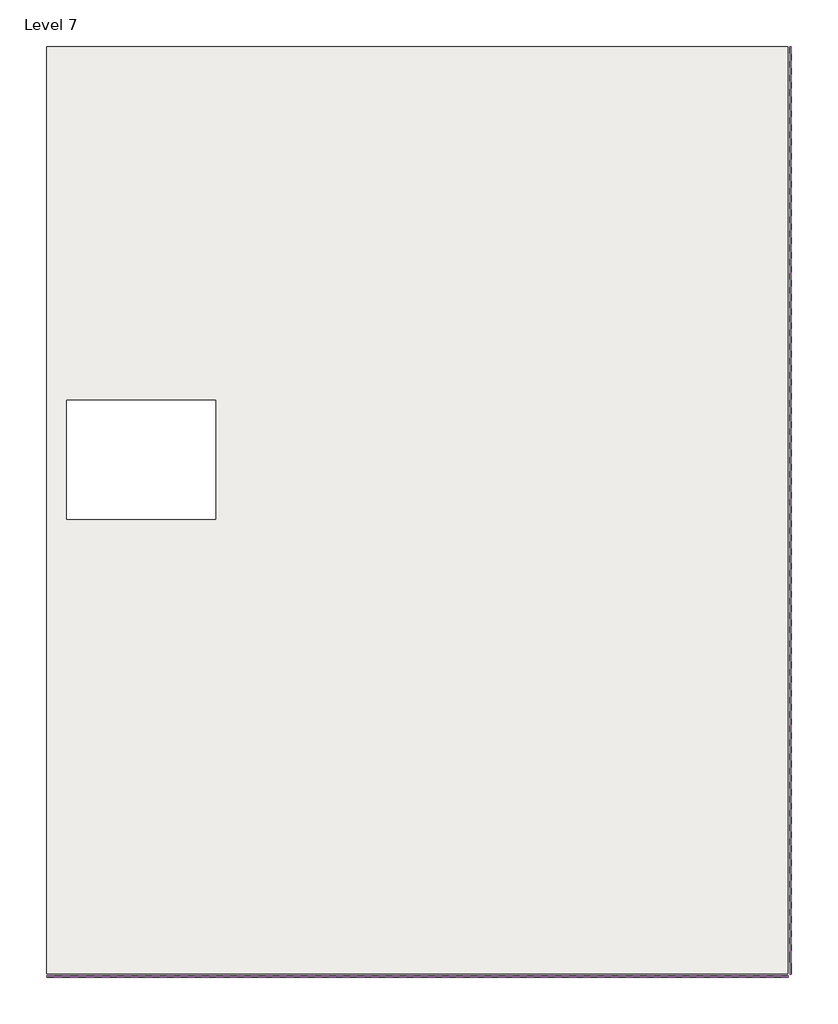
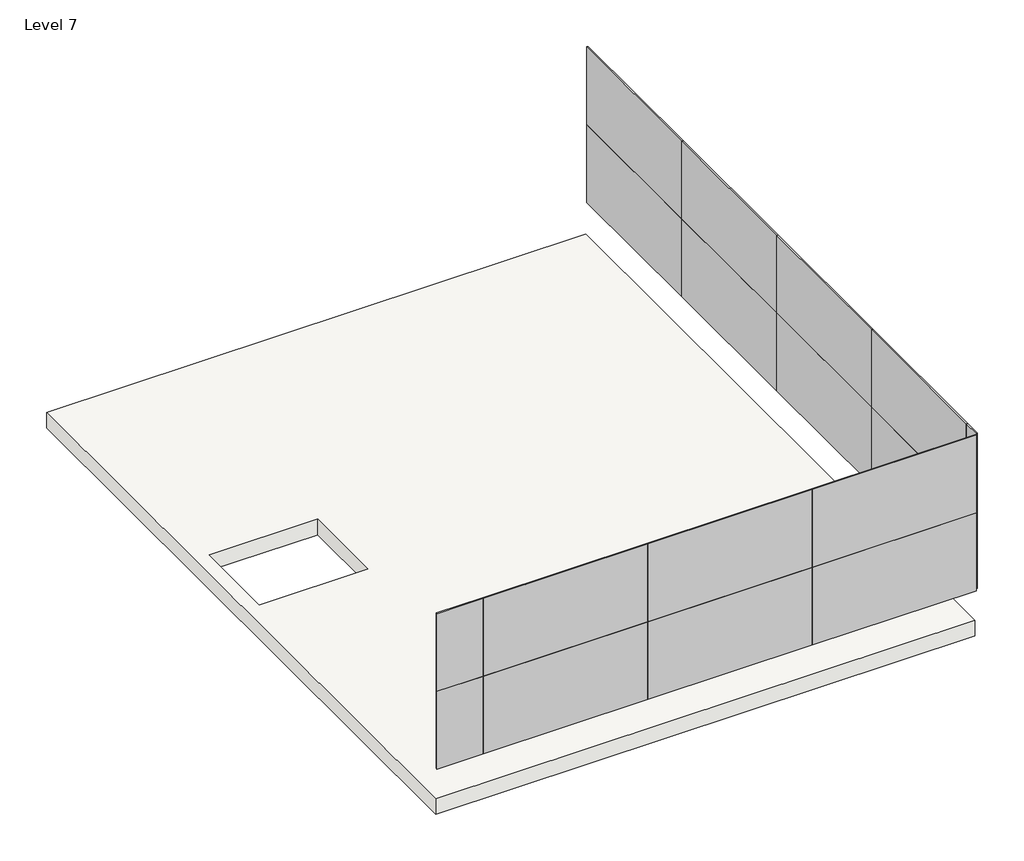
# One storey: 18 plates, 1 slab.
"""IFC4 building model written with IfcOpenShell, lengths in millimetres."""

import ifcopenshell
import ifcopenshell.guid

model = None  # the IFC model being written
_history = None  # IfcOwnerHistory: only IFC2X3 demands one
_inside = {}  # id of a spatial element -> (the spatial element, [elements in it])
_under = {}  # id of a project, library or spatial element -> (it, [spatial elements below it])
_declared = {}  # id of a project -> (the project, [libraries it declares])
_typed = {}  # id of a type object -> (the type object, [elements of that type])
_made_of = {}  # id of a material, layer set ... -> (it, [elements and type objects made of it])


def new_model(schema):
    """Start an empty IFC model of exactly this schema.

    Asked for "IFC4X3", IfcOpenShell would pick the latest addendum, in which some entities
    have other attributes; the version numbers below select the first issue.
    IFC2X3 requires an IfcOwnerHistory on every rooted entity: one is made here for all.
    """
    global model, _history
    if schema == "IFC4X3":
        model = ifcopenshell.file(schema_version=(4, 3, 0, 0))
    else:
        model = ifcopenshell.file(schema=schema)
    _inside.clear()
    _under.clear()
    _declared.clear()
    _typed.clear()
    _made_of.clear()
    _history = None
    if model.schema == "IFC2X3":
        org = make("IfcOrganization", Name="unknown")
        user = make(
            "IfcPersonAndOrganization",
            ThePerson=make("IfcPerson", FamilyName="unknown"),
            TheOrganization=org,
        )
        app = make(
            "IfcApplication",
            ApplicationDeveloper=org,
            Version="unknown",
            ApplicationFullName="unknown",
            ApplicationIdentifier="unknown",
        )
        _history = make(
            "IfcOwnerHistory",
            OwningUser=user,
            OwningApplication=app,
            ChangeAction="ADDED",
            CreationDate=0,
        )
    return model


def make(cls, **values):
    """One entity of the class cls with the attributes given. An attribute that is None is left unset."""
    return model.create_entity(
        cls, **{name: value for name, value in values.items() if value is not None}
    )


def rooted(cls, **values):
    """An entity with a GlobalId (a new one), such as an element, a storey or a relation."""
    return make(cls, GlobalId=ifcopenshell.guid.new(), OwnerHistory=_history, **values)


def si_unit(unit_type, name, prefix=None):
    """IfcSIUnit, for example si_unit("LENGTHUNIT", "METRE", prefix="MILLI")."""
    return make("IfcSIUnit", UnitType=unit_type, Prefix=prefix, Name=name)


def assignment(units):
    """IfcUnitAssignment: the units of a project."""
    return None if units is None else make("IfcUnitAssignment", Units=units)


def point(xyz):
    """IfcCartesianPoint."""
    return None if xyz is None else make("IfcCartesianPoint", Coordinates=xyz)


def direction(xyz):
    """IfcDirection."""
    return None if xyz is None else make("IfcDirection", DirectionRatios=xyz)


def frame(location, z_axis=None, x_axis=None):
    """IfcAxis2Placement3D, a coordinate frame: its origin and axes. An axis left out is left unset."""
    return make(
        "IfcAxis2Placement3D",
        Location=point(location),
        Axis=direction(z_axis),
        RefDirection=direction(x_axis),
    )


def origin():
    """The frame at (0, 0, 0) with its axes left unset."""
    return frame((0.0, 0.0, 0.0))


def origin_with_axes():
    """The frame at (0, 0, 0) with the z axis (0, 0, 1) and the x axis (1, 0, 0) written out."""
    return frame((0.0, 0.0, 0.0), z_axis=(0.0, 0.0, 1.0), x_axis=(1.0, 0.0, 0.0))


def place(relative_to, where):
    """IfcLocalPlacement: puts the frame where relative to a parent placement (None: the world)."""
    return make(
        "IfcLocalPlacement", PlacementRelTo=relative_to, RelativePlacement=where
    )


def context(
    kind, dimensions, precision=None, world=None, true_north=None, identifier=None
):
    """IfcGeometricRepresentationContext, for example the 3D "Model" context."""
    return make(
        "IfcGeometricRepresentationContext",
        ContextIdentifier=identifier,
        ContextType=kind,
        CoordinateSpaceDimension=dimensions,
        Precision=precision,
        WorldCoordinateSystem=world,
        TrueNorth=true_north,
    )


def project(units=None, contexts=None):
    """IfcProject with its units and contexts."""
    return rooted(
        "IfcProject",
        Name="project",
        RepresentationContexts=contexts,
        UnitsInContext=assignment(units),
    )


def spatial(cls, under=None, at=None, **own):
    """A site, building, storey or space (cls), placed at a placement, below another one or the project."""
    s = rooted(cls, ObjectPlacement=at, **own)
    if under is not None:
        _under.setdefault(under.id(), (under, []))[1].append(s)
    return s


def polyline(points):
    """IfcPolyline through the points."""
    return make("IfcPolyline", Points=[point(p) for p in points])


def outline(outer, holes=None, kind="AREA"):
    """IfcArbitraryClosedProfileDef: a profile drawn as a closed curve; with holes, ...WithVoids."""
    if holes is None:
        return make("IfcArbitraryClosedProfileDef", ProfileType=kind, OuterCurve=outer)
    return make(
        "IfcArbitraryProfileDefWithVoids",
        ProfileType=kind,
        OuterCurve=outer,
        InnerCurves=holes,
    )


def extrude(swept, where, along, depth):
    """IfcExtrudedAreaSolid: the profile swept, set in the frame where, extruded along a direction by depth."""
    return make(
        "IfcExtrudedAreaSolid",
        SweptArea=swept,
        Position=where,
        ExtrudedDirection=direction(along),
        Depth=depth,
    )


def shape(context_of_items, identifier, shape_type, items):
    """IfcShapeRepresentation: the items that make up one representation, for example the "Body"."""
    return make(
        "IfcShapeRepresentation",
        ContextOfItems=context_of_items,
        RepresentationIdentifier=identifier,
        RepresentationType=shape_type,
        Items=items,
    )


def source(mapping_origin, context_of_items, identifier, shape_type, items):
    """IfcRepresentationMap: a shape defined once, which mapped items show again and again."""
    return make(
        "IfcRepresentationMap",
        MappingOrigin=mapping_origin,
        MappedRepresentation=shape(context_of_items, identifier, shape_type, items),
    )


def transform(
    local_origin,
    x_axis=None,
    y_axis=None,
    z_axis=None,
    scale=None,
    scale2=None,
    scale3=None,
    uniform=True,
):
    """IfcCartesianTransformationOperator3D, or its non-uniform kind. x_axis, y_axis, z_axis: its Axis1, 2, 3."""
    if uniform:
        return make(
            "IfcCartesianTransformationOperator3D",
            Axis1=direction(x_axis),
            Axis2=direction(y_axis),
            LocalOrigin=point(local_origin),
            Scale=scale,
            Axis3=direction(z_axis),
        )
    return make(
        "IfcCartesianTransformationOperator3DnonUniform",
        Axis1=direction(x_axis),
        Axis2=direction(y_axis),
        LocalOrigin=point(local_origin),
        Scale=scale,
        Axis3=direction(z_axis),
        Scale2=scale2,
        Scale3=scale3,
    )


def mapped(mapping_source, mapping_target):
    """IfcMappedItem: shows the shape of a source again, moved by a transform."""
    return make(
        "IfcMappedItem", MappingSource=mapping_source, MappingTarget=mapping_target
    )


def made_of(thing, what):
    """Note that an element or type object is made of a material, layer set ...; save() writes the relation."""
    if what is not None:
        _made_of.setdefault(what.id(), (what, []))[1].append(thing)
    return thing


def element(
    cls,
    number,
    at=None,
    inside=None,
    cuts=None,
    type_object=None,
    material=None,
    context=None,
    identifier="Body",
    shape_type=None,
    held_by="IfcProductDefinitionShape",
    body=None,
    shapes=None,
    **own,
):
    """One element of the class cls, such as IfcWall. Its Tag is "e" and its number.

    at: its placement. inside: the storey or other place that contains it. cuts: it is an
    opening in that element (IfcRelVoidsElement). A single representation is given by context,
    identifier, shape_type and body (its items); several are given by shapes. held_by: the class
    of the entity that holds the representations. save() writes the other relations.
    """
    e = rooted(cls, Tag="e%d" % number, ObjectPlacement=at, **own)
    if body is not None:
        shapes = [shape(context, identifier, shape_type, body)]
    if shapes is not None:
        e.Representation = make(held_by, Representations=shapes)
    if inside is not None:
        _inside.setdefault(inside.id(), (inside, []))[1].append(e)
    if cuts is not None:
        rooted(
            "IfcRelVoidsElement", RelatingBuildingElement=cuts, RelatedOpeningElement=e
        )
    if type_object is not None:
        _typed.setdefault(type_object.id(), (type_object, []))[1].append(e)
    return made_of(e, material)


def aggregate(whole, parts):
    """IfcRelAggregates: a whole, such as a stair, and the parts it consists of."""
    return rooted("IfcRelAggregates", RelatingObject=whole, RelatedObjects=parts)


def save(model, path):
    """Write the relations noted so far, then the file.

    IfcRelAggregates (storeys below a building ...), IfcRelContainedInSpatialStructure (elements
    in a storey), IfcRelDefinesByType, IfcRelAssociatesMaterial and IfcRelDeclares: one each for
    every whole, place, type object, material and project.
    """
    for whole, parts in _under.values():
        aggregate(whole, parts)
    for where, things in _inside.values():
        rooted(
            "IfcRelContainedInSpatialStructure",
            RelatedElements=things,
            RelatingStructure=where,
        )
    for kind, things in _typed.values():
        rooted("IfcRelDefinesByType", RelatedObjects=things, RelatingType=kind)
    for what, things in _made_of.values():
        rooted("IfcRelAssociatesMaterial", RelatedObjects=things, RelatingMaterial=what)
    for by, libraries in _declared.values():
        rooted("IfcRelDeclares", RelatingContext=by, RelatedDefinitions=libraries)
    model.write(path)


def system_panel_glazed_1e57f9bb(model_context):
    return source(origin(), model_context, "Body", "SweptSolid", [
        extrude(outline(polyline([(1524.0000002, 19.05), (-1524.0000002, 19.05), (-1524.0000002, 44.45), (1524.0000002, 44.45), (1524.0000002, 19.05)])), origin_with_axes(), (0.0, 0.0, 1.0), 1524.0),
    ])


def system_panel_glazed_ccfd9adb(model_context):
    return source(origin(), model_context, "Body", "SweptSolid", [
        extrude(outline(polyline([(427.9999998, 19.05), (-427.9999998, 19.05), (-427.9999998, 44.45), (427.9999998, 44.45), (427.9999998, 19.05)])), origin_with_axes(), (0.0, 0.0, 1.0), 1524.0),
    ])


def system_panel_glazed_88f24eba(model_context):
    return source(origin(), model_context, "Body", "SweptSolid", [
        extrude(outline(polyline([(153.9999998, 19.05), (-153.9999998, 19.05), (-153.9999998, 44.45), (153.9999998, 44.45), (153.9999998, 19.05)])), origin_with_axes(), (0.0, 0.0, 1.0), 1524.0),
    ])


model = new_model("IFC4")

# Units and contexts
model_context = context("Model", 3, world=origin())
ifc_project = project(units=[si_unit("LENGTHUNIT", "METRE", prefix="MILLI")], contexts=[model_context])

# Site, building, storey
site = spatial("IfcSite", under=ifc_project)
building = spatial("IfcBuilding", under=site)
storey = spatial("IfcBuildingStorey", under=building, Name="Level 7", Elevation=19200.0)

# Plates
placement = place(None, origin())
system_panel_glazed_shape = system_panel_glazed_1e57f9bb(model_context)
element("IfcPlate", 1, ObjectType="System Panel : Glazed", at=placement, inside=storey, context=model_context, shape_type="MappedRepresentation", body=[
    mapped(system_panel_glazed_shape, transform((2137.6340362, 1399.6955828, 19812.0), x_axis=(-1.0, 0.0, 0.0), y_axis=(0.0, -1.0, 0.0), z_axis=(0.0, 0.0, 1.0))),
])
element("IfcPlate", 2, ObjectType="System Panel : Glazed", at=placement, inside=storey, context=model_context, shape_type="MappedRepresentation", body=[
    mapped(system_panel_glazed_shape, transform((-910.3659639, 1399.6955828, 19812.0), x_axis=(-1.0, 0.0, 0.0), y_axis=(0.0, -1.0, 0.0), z_axis=(0.0, 0.0, 1.0))),
])
element("IfcPlate", 3, ObjectType="System Panel : Glazed", at=placement, inside=storey, context=model_context, shape_type="MappedRepresentation", body=[
    mapped(system_panel_glazed_shape, transform((-3958.3659639, 1399.6955828, 19812.0), x_axis=(-1.0, 0.0, 0.0), y_axis=(0.0, -1.0, 0.0), z_axis=(0.0, 0.0, 1.0))),
])
element("IfcPlate", 4, ObjectType="System Panel : Glazed", at=placement, inside=storey, context=model_context, shape_type="MappedRepresentation", body=[
    mapped(system_panel_glazed_shape, transform((2137.6340362, 1399.6955828, 21336.0), x_axis=(-1.0, 0.0, 0.0), y_axis=(0.0, -1.0, 0.0), z_axis=(0.0, 0.0, 1.0))),
])
element("IfcPlate", 5, ObjectType="System Panel : Glazed", at=placement, inside=storey, context=model_context, shape_type="MappedRepresentation", body=[
    mapped(system_panel_glazed_shape, transform((-910.3659639, 1399.6955828, 21336.0), x_axis=(-1.0, 0.0, 0.0), y_axis=(0.0, -1.0, 0.0), z_axis=(0.0, 0.0, 1.0))),
])
element("IfcPlate", 6, ObjectType="System Panel : Glazed", at=placement, inside=storey, context=model_context, shape_type="MappedRepresentation", body=[
    mapped(system_panel_glazed_shape, transform((-3958.3659639, 1399.6955828, 21336.0), x_axis=(-1.0, 0.0, 0.0), y_axis=(0.0, -1.0, 0.0), z_axis=(0.0, 0.0, 1.0))),
])
element("IfcPlate", 7, ObjectType="System Panel : Glazed", at=placement, inside=storey, context=model_context, shape_type="MappedRepresentation", body=[
    mapped(system_panel_glazed_shape, transform((3661.6340364, 12375.6955827, 19812.0), x_axis=(0.0, -1.0, 0.0), y_axis=(1.0, 0.0, 0.0), z_axis=(0.0, 0.0, 1.0))),
])
element("IfcPlate", 8, ObjectType="System Panel : Glazed", at=placement, inside=storey, context=model_context, shape_type="MappedRepresentation", body=[
    mapped(system_panel_glazed_shape, transform((3661.6340364, 9327.6955825, 19812.0), x_axis=(0.0, -1.0, 0.0), y_axis=(1.0, 0.0, 0.0), z_axis=(0.0, 0.0, 1.0))),
])
element("IfcPlate", 9, ObjectType="System Panel : Glazed", at=placement, inside=storey, context=model_context, shape_type="MappedRepresentation", body=[
    mapped(system_panel_glazed_shape, transform((3661.6340364, 6279.6955825, 19812.0), x_axis=(0.0, -1.0, 0.0), y_axis=(1.0, 0.0, 0.0), z_axis=(0.0, 0.0, 1.0))),
])
element("IfcPlate", 10, ObjectType="System Panel : Glazed", at=placement, inside=storey, context=model_context, shape_type="MappedRepresentation", body=[
    mapped(system_panel_glazed_shape, transform((3661.6340364, 3231.6955825, 19812.0), x_axis=(0.0, -1.0, 0.0), y_axis=(1.0, 0.0, 0.0), z_axis=(0.0, 0.0, 1.0))),
])
element("IfcPlate", 11, ObjectType="System Panel : Glazed", at=placement, inside=storey, context=model_context, shape_type="MappedRepresentation", body=[
    mapped(system_panel_glazed_shape, transform((3661.6340364, 12375.6955827, 21336.0), x_axis=(0.0, -1.0, 0.0), y_axis=(1.0, 0.0, 0.0), z_axis=(0.0, 0.0, 1.0))),
])
element("IfcPlate", 12, ObjectType="System Panel : Glazed", at=placement, inside=storey, context=model_context, shape_type="MappedRepresentation", body=[
    mapped(system_panel_glazed_shape, transform((3661.6340364, 9327.6955825, 21336.0), x_axis=(0.0, -1.0, 0.0), y_axis=(1.0, 0.0, 0.0), z_axis=(0.0, 0.0, 1.0))),
])
element("IfcPlate", 13, ObjectType="System Panel : Glazed", at=placement, inside=storey, context=model_context, shape_type="MappedRepresentation", body=[
    mapped(system_panel_glazed_shape, transform((3661.6340364, 6279.6955825, 21336.0), x_axis=(0.0, -1.0, 0.0), y_axis=(1.0, 0.0, 0.0), z_axis=(0.0, 0.0, 1.0))),
])
element("IfcPlate", 14, ObjectType="System Panel : Glazed", at=placement, inside=storey, context=model_context, shape_type="MappedRepresentation", body=[
    mapped(system_panel_glazed_shape, transform((3661.6340364, 3231.6955825, 21336.0), x_axis=(0.0, -1.0, 0.0), y_axis=(1.0, 0.0, 0.0), z_axis=(0.0, 0.0, 1.0))),
])
system_panel_glazed_2_shape = system_panel_glazed_ccfd9adb(model_context)
element("IfcPlate", 15, ObjectType="System Panel : Glazed", at=placement, inside=storey, context=model_context, shape_type="MappedRepresentation", body=[
    mapped(system_panel_glazed_2_shape, transform((-5910.3659638, 1399.6955828, 19812.0), x_axis=(-1.0, 0.0, 0.0), y_axis=(0.0, -1.0, 0.0), z_axis=(0.0, 0.0, 1.0))),
])
element("IfcPlate", 16, ObjectType="System Panel : Glazed", at=placement, inside=storey, context=model_context, shape_type="MappedRepresentation", body=[
    mapped(system_panel_glazed_2_shape, transform((-5910.3659638, 1399.6955828, 21336.0), x_axis=(-1.0, 0.0, 0.0), y_axis=(0.0, -1.0, 0.0), z_axis=(0.0, 0.0, 1.0))),
])
system_panel_glazed_3_shape = system_panel_glazed_88f24eba(model_context)
element("IfcPlate", 17, ObjectType="System Panel : Glazed", at=placement, inside=storey, context=model_context, shape_type="MappedRepresentation", body=[
    mapped(system_panel_glazed_3_shape, transform((3661.6340364, 1553.6955827, 19812.0), x_axis=(0.0, -1.0, 0.0), y_axis=(1.0, 0.0, 0.0), z_axis=(0.0, 0.0, 1.0))),
])
element("IfcPlate", 18, ObjectType="System Panel : Glazed", at=placement, inside=storey, context=model_context, shape_type="MappedRepresentation", body=[
    mapped(system_panel_glazed_3_shape, transform((3661.6340364, 1553.6955827, 21336.0), x_axis=(0.0, -1.0, 0.0), y_axis=(1.0, 0.0, 0.0), z_axis=(0.0, 0.0, 1.0))),
])

# Slab
element("IfcSlab", 19, ObjectType="Generic - 12\"", at=placement, inside=storey, context=model_context, shape_type="SweptSolid", body=[
    extrude(outline(polyline([(-6335.3659636, 1402.6955828), (-6335.3659636, 13896.6955828), (3658.6340364, 13896.6955828), (3658.6340364, 1402.6955828), (-6335.3659636, 1402.6955828)]), holes=[polyline([(-4059.8993101, 7527.9023719), (-4059.8993101, 9133.9023719), (-6065.8993101, 9133.9023719), (-6065.8993101, 7527.9023719), (-4059.8993101, 7527.9023719)])]), frame((0.0, 0.0, 18895.2), z_axis=(0.0, 0.0, 1.0), x_axis=(1.0, 0.0, 0.0)), (0.0, 0.0, 1.0), 304.8),
])

save(model, "model.ifc")

# Revit data of these elements
# Type "System Panel : Glazed"
#   Construction Type Id = "GSP4R"
#   Analytic Construction = "1/8 in Pilkington single glazing"
#   Visual Light Transmittance = 0.9
#   Solar Heat Gain Coefficient = 0.86
#   Heat Transfer Coefficient (U) = 6.7069 W/(m²·K)
# Type "Generic - 12\""
#   Assembly Code = "B1010"
#   Function = 0
#   Layers, outside or top first: 0.3048 m no material (function 1)
# Elements 1, 2, 3, 4, 5, 6, 7, 8, 9, 10, 11, 12, 13, 14, 15, 16, 17, 18 (IfcPlate, "System Panel : Glazed")
#   Phase Created = New Construction
#   Materials on its faces: "Glass"
# Element 19 (IfcSlab, "Generic - 12\"")
#   built-in parameter 1001955 = -1.5708 (stored number, unit not read)
#   Height Offset From Level = 0.00 m
#   Phase Created = New Construction
#   Materials on its faces: "Default Floor"
# Materials
#   "Glass": class "Glass", colour RGB 0 128 192, transparency 0.75, Description = "Soda Lime Glass", Cost = 0
#   "Default Floor": class "Miscellaneous", colour RGB 128 128 128, transparency 0, Cost = 0
